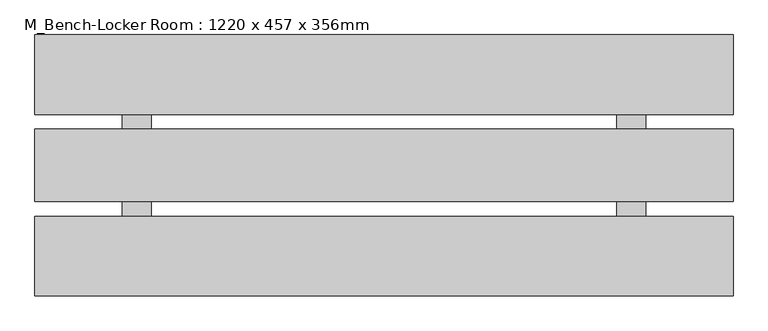
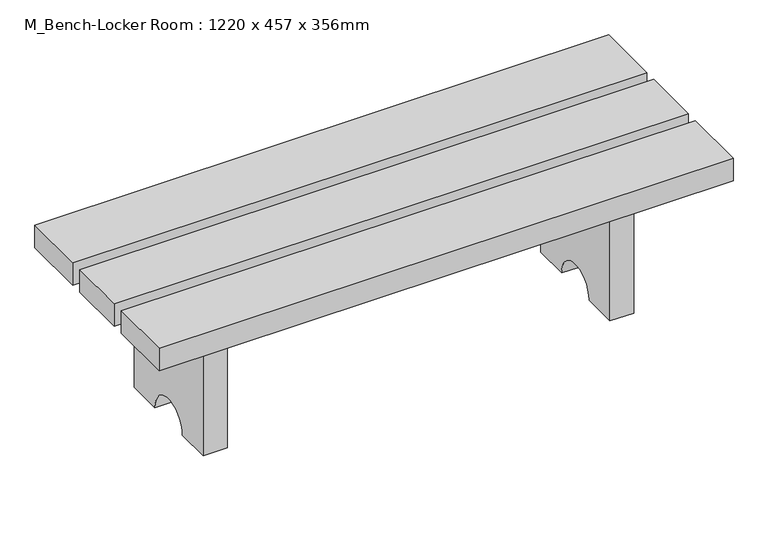
"""IFC4 building model written with IfcOpenShell, lengths in millimetres: furniture geometry, M_Bench-Locker Room : 1220 x 457 x 356mm."""

from ifc_helpers import new_model, si_unit, point, frame, frame_2d, origin, place, context, project, spatial, polyline, circle_curve, trimmed, segment, composite_curve, outline, extrude, source, transform, mapped, element, save


def m_bench_locker_room_1220_x_457_x_356mm_af128f29(model_context):
    return source(origin(), model_context, "Body", "SweptSolid", [
        extrude(outline(composite_curve([segment(polyline([(-307.6147541, 0.0), (-307.6147541, 305.2), (-53.8147541, 305.2), (-53.8147541, 0.0), (-130.0147541, 0.0)]), True, "CONTINUOUS"), segment(trimmed(circle_curve(frame_2d((-180.7147541, 0.0)), 50.7), [point((-130.0147541, 0.0))], [point((-231.4147541, 0.0))], True, "CARTESIAN"), True, "CONTINUOUS"), segment(polyline([(-231.4147541, 0.0), (-307.6147541, 0.0)]), True, "CONTINUOUS")], self_intersect=False)), frame((251.4852459, 0.0, 0.0), z_axis=(1.0, 0.0, 0.0), x_axis=(0.0, 1.0, 0.0)), (0.0, 0.0, 1.0), 50.8),
        extrude(outline(composite_curve([segment(polyline([(-53.8147541, 0.0), (-130.0147541, 0.0)]), True, "CONTINUOUS"), segment(trimmed(circle_curve(frame_2d((-180.7147541, 0.0)), 50.7), [point((-130.0147541, 0.0))], [point((-231.4147541, 0.0))], True, "CARTESIAN"), True, "CONTINUOUS"), segment(polyline([(-231.4147541, 0.0), (-307.6147541, 0.0), (-307.6147541, 305.2), (-53.8147541, 305.2), (-53.8147541, 0.0)]), True, "CONTINUOUS")], self_intersect=False)), frame((-612.9147541, 0.0, 0.0), z_axis=(1.0, 0.0, 0.0), x_axis=(0.0, 1.0, 0.0)), (0.0, 0.0, 1.0), 50.8),
        extrude(outline(polyline([(454.6852459, 47.7852459), (454.6852459, -91.8480874), (-765.3147541, -91.8480874), (-765.3147541, 47.7852459), (454.6852459, 47.7852459)])), frame((0.0, 0.0, 305.2), z_axis=(0.0, 0.0, 1.0), x_axis=(1.0, 0.0, 0.0)), (0.0, 0.0, 1.0), 50.8),
        extrude(outline(polyline([(454.6852459, -409.2147541), (-765.3147541, -409.2147541), (-765.3147541, -269.5814208), (454.6852459, -269.5814208), (454.6852459, -409.2147541)])), frame((0.0, 0.0, 305.2), z_axis=(0.0, 0.0, 1.0), x_axis=(1.0, 0.0, 0.0)), (0.0, 0.0, 1.0), 50.8),
        extrude(outline(polyline([(454.6852459, -117.2480874), (454.6852459, -244.1814208), (-765.3147541, -244.1814208), (-765.3147541, -117.2480874), (454.6852459, -117.2480874)])), frame((0.0, 0.0, 305.2), z_axis=(0.0, 0.0, 1.0), x_axis=(1.0, 0.0, 0.0)), (0.0, 0.0, 1.0), 50.8),
    ])


if __name__ == "__main__":
    model = new_model("IFC4")
    model_context = context("Model", 3, world=origin())
    ifc_project = project(units=[si_unit("LENGTHUNIT", "METRE", prefix="MILLI")], contexts=[model_context])
    site = spatial("IfcSite", under=ifc_project)
    building = spatial("IfcBuilding", under=site)
    placement = place(None, origin())
    m_bench_locker_room_1220_x_457_x_356mm_shape = m_bench_locker_room_1220_x_457_x_356mm_af128f29(model_context)
    element("IfcFurniture", 1, ObjectType="M_Bench-Locker Room : 1220 x 457 x 356mm", at=placement, inside=building, context=model_context, shape_type="MappedRepresentation", body=[
        mapped(m_bench_locker_room_1220_x_457_x_356mm_shape, transform((0.0, 0.0, 0.0), x_axis=(1.0, 0.0, 0.0), y_axis=(0.0, 1.0, 0.0), z_axis=(0.0, 0.0, 1.0))),
    ])
    save(model, "model.ifc")

# Revit data of these elements
# Type "M_Bench-Locker Room : 1220 x 457 x 356mm"
#   Depth = 0.457 m
#   Height = 0.356 m
#   Width = 1.22 m
#   Bench Material = Cherry
#   Default Elevation = 0
# Element 1 (IfcFurniture, "M_Bench-Locker Room : 1220 x 457 x 356mm")
#   Materials on its faces: "Cherry"
# Materials
#   "Cherry": class "Wood", colour RGB 157 77 38, transparency 0, Description = "Prunus Serotina", Cost = 0
